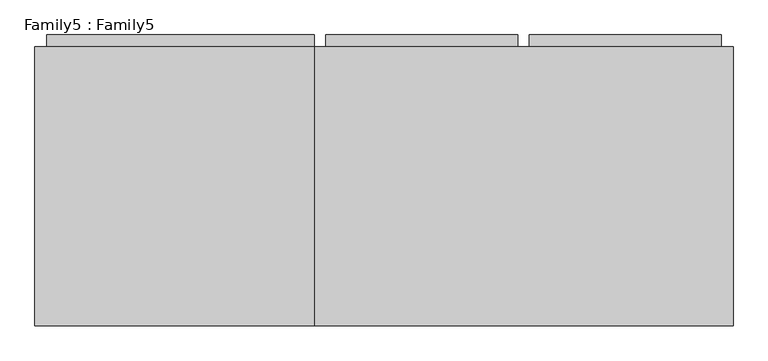
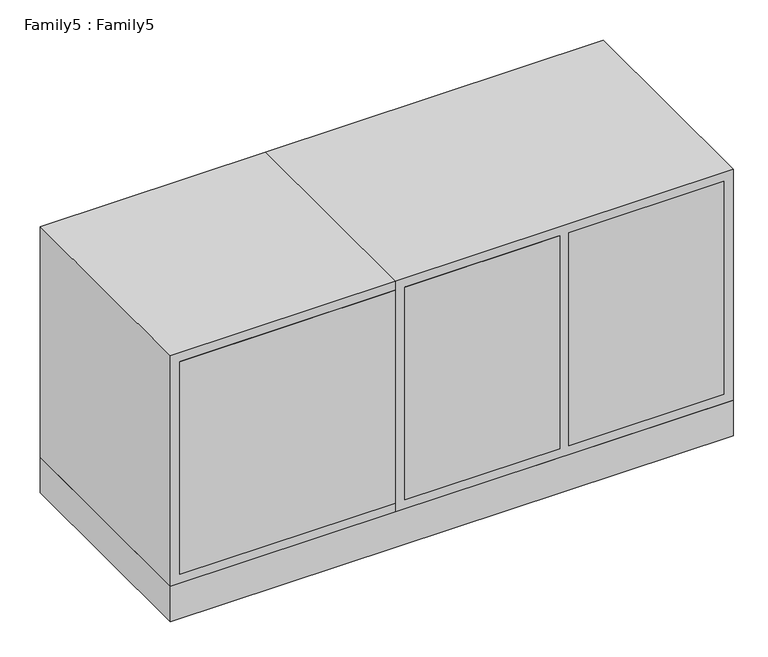
"""IFC4 building model written with IfcOpenShell, lengths in millimetres: proxy geometry, Family5 : Family5."""

from ifc_helpers import new_model, si_unit, frame, origin, place, context, project, spatial, polyline, outline, extrude, source, transform, mapped, element, save


def family5_family5_76c3a8f9(model_context):
    return source(origin(), model_context, "Body", "SweptSolid", [
        extrude(outline(polyline([(-1041.4, 685.8), (-457.2, 685.8), (-457.2, 50.8), (-1041.4, 50.8), (-1041.4, 685.8)])), frame((0.0, 0.0, 1574.244413), z_axis=(0.0, 0.0, 1.0), x_axis=(1.0, 0.0, 0.0)), (0.0, 0.0, 1.0), 609.6),
        extrude(outline(polyline([(12.7, 685.8), (431.8, 685.8), (431.8, 50.8), (12.7, 50.8), (12.7, 685.8)])), frame((0.0, 0.0, 1574.244413), z_axis=(0.0, 0.0, 1.0), x_axis=(1.0, 0.0, 0.0)), (0.0, 0.0, 1.0), 609.6),
        extrude(outline(polyline([(-431.8, 685.8), (-12.7, 685.8), (-12.7, 50.8), (-431.8, 50.8), (-431.8, 685.8)])), frame((0.0, 0.0, 1574.244413), z_axis=(0.0, 0.0, 1.0), x_axis=(1.0, 0.0, 0.0)), (0.0, 0.0, 1.0), 609.6),
        extrude(outline(polyline([(-1066.8, 660.4), (-457.2, 660.4), (-457.2, 50.8), (-1066.8, 50.8), (-1066.8, 660.4)])), frame((0.0, 0.0, 1548.844413), z_axis=(0.0, 0.0, 1.0), x_axis=(1.0, 0.0, 0.0)), (0.0, 0.0, 1.0), 660.4),
        extrude(outline(polyline([(-457.2, 660.4), (457.2, 660.4), (457.2, 50.8), (-457.2, 50.8), (-457.2, 660.4)])), frame((0.0, 0.0, 1548.844413), z_axis=(0.0, 0.0, 1.0), x_axis=(1.0, 0.0, 0.0)), (0.0, 0.0, 1.0), 660.4),
        extrude(outline(polyline([(-1066.8, 660.4), (457.2, 660.4), (457.2, 50.8), (-1066.8, 50.8), (-1066.8, 660.4)])), frame((0.0, 0.0, 1447.244413), z_axis=(0.0, 0.0, 1.0), x_axis=(1.0, 0.0, 0.0)), (0.0, 0.0, 1.0), 101.6),
    ])


if __name__ == "__main__":
    model = new_model("IFC4")
    model_context = context("Model", 3, world=origin())
    ifc_project = project(units=[si_unit("LENGTHUNIT", "METRE", prefix="MILLI")], contexts=[model_context])
    site = spatial("IfcSite", under=ifc_project)
    building = spatial("IfcBuilding", under=site)
    placement = place(None, origin())
    family5_family5_shape = family5_family5_76c3a8f9(model_context)
    element("IfcBuildingElementProxy", 1, Name="Family5 : Family5", ObjectType="Family5 : Family5", at=placement, inside=building, context=model_context, shape_type="MappedRepresentation", body=[
        mapped(family5_family5_shape, transform((0.0, 0.0, 0.0), x_axis=(1.0, 0.0, 0.0), y_axis=(0.0, 1.0, 0.0), z_axis=(0.0, 0.0, 1.0))),
    ])
    save(model, "model.ifc")

# Revit data of these elements
# Type "Family5 : Family5"
#   strip depth = 0' - 1"
#   drawer depth = 2' - 1"
#   cabinet depth = 2' - 0"
#   bottom thickness = 0' - 4"
#   Total height = 2' - 6"
#   Default Elevation = 0
